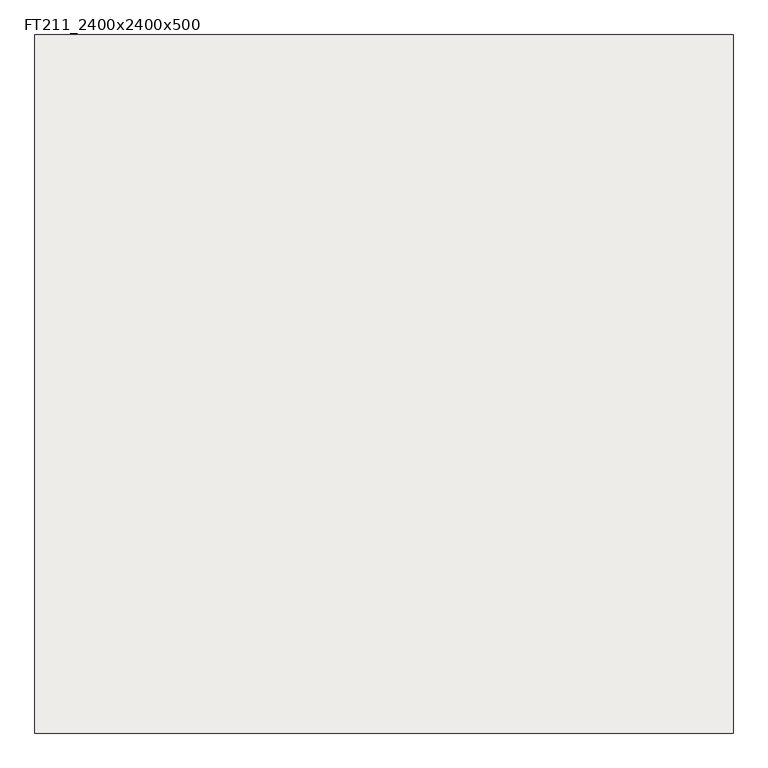
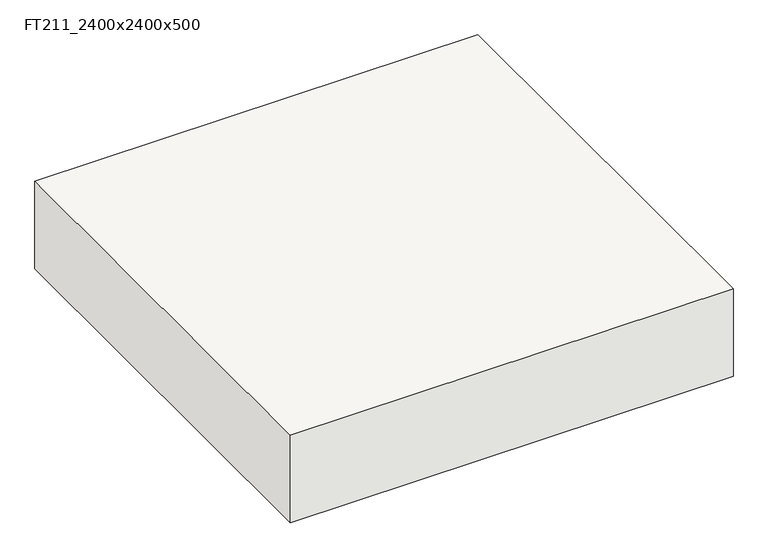
"""IFC4 building model written with IfcOpenShell, lengths in millimetres: slab geometry, FT211-Footing-Rectangular_더미삭제 : FT211_2400x2400x500."""

from ifc_helpers import new_model, si_unit, frame, origin, place, context, project, spatial, polyline, outline, extrude, source, transform, mapped, element, save


def ft211_2400x2400x500_5fe39465(model_context):
    return source(origin(), model_context, "Body", "SweptSolid", [
        extrude(outline(polyline([(1200.0, 1200.0), (1200.0, -1200.0), (-1200.0, -1200.0), (-1200.0, 1200.0), (1200.0, 1200.0)])), frame((0.0, 0.0, -500.0), z_axis=(0.0, 0.0, 1.0), x_axis=(1.0, 0.0, 0.0)), (0.0, 0.0, 1.0), 500.0),
    ])


if __name__ == "__main__":
    model = new_model("IFC4")
    model_context = context("Model", 3, world=origin())
    ifc_project = project(units=[si_unit("LENGTHUNIT", "METRE", prefix="MILLI")], contexts=[model_context])
    site = spatial("IfcSite", under=ifc_project)
    building = spatial("IfcBuilding", under=site)
    placement = place(None, origin())
    ft211_2400x2400x500_shape = ft211_2400x2400x500_5fe39465(model_context)
    element("IfcSlab", 1, ObjectType="FT211-Footing-Rectangular_더미삭제 : FT211_2400x2400x500", at=placement, inside=building, context=model_context, shape_type="MappedRepresentation", body=[
        mapped(ft211_2400x2400x500_shape, transform((0.0, 0.0, 0.0), x_axis=(1.0, 0.0, 0.0), y_axis=(0.0, 1.0, 0.0), z_axis=(0.0, 0.0, 1.0))),
    ])
    save(model, "model.ifc")

# Revit data of these elements
# Type "FT211-Footing-Rectangular_더미삭제 : FT211_2400x2400x500"
#   Top bar = "D25@300"
#   Description = "UG Shallow Foundation"
#   Bottom bar = "D20@300"
#   Width = 2400 mm
#   Length = 2400 mm
#   Foundation Thickness = 500 mm
#   Structural Material [instance default] = A03AC032-00007_Structural Concrete_Type1_25MPa-30Mpa
#   Assembly Code = ""
# Element 1 (IfcSlab, "FT211-Footing-Rectangular_더미삭제 : FT211_2400x2400x500")
#   Materials on its faces: "A03AC032-00007_Structural Concrete_Type1_25MPa-30Mpa"
# Materials
#   "A03AC032-00007_Structural Concrete_Type1_25MPa-30Mpa": class "Concrete", colour RGB 176 176 176, transparency 0, Keynote = "09910.A1", Description = "Reinf. Conc.", W00) Work Master Code = "A03AC032-00007", W01) Work Master_Lv1 = "Concrete Work", W02) Work Master_Lv2 = "Substructure Work", W03) Work Master_Spec.1 = "Structural Concrete", W04) Work Master_Spec.2 = "Cement Type-1", W05) Work Master_Spec.3 = "25MPa < F'c (Cylinder Strength) ≤ 30MPa", Cost = 0
